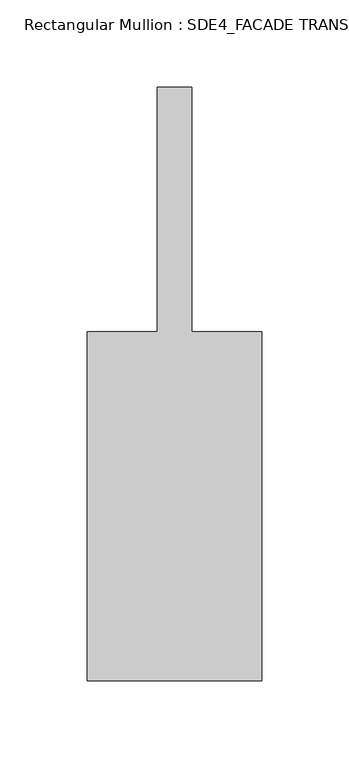
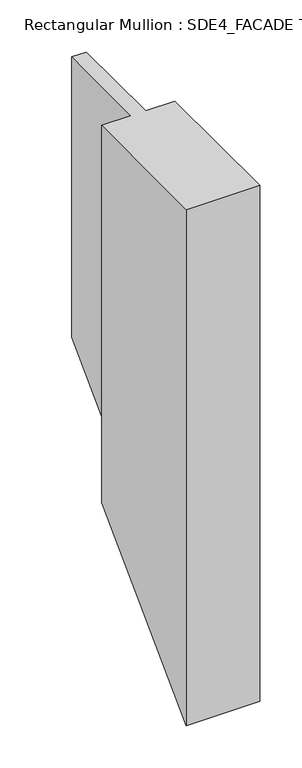
"""IFC4 building model written with IfcOpenShell, lengths in millimetres: member geometry, Rectangular Mullion : SDE4_FACADE TRANSOM TYPE 1."""

from ifc_helpers import new_model, si_unit, origin, place, context, project, spatial, faceted_brep, source, transform, mapped, element, save


def rectangular_mullion_sde4_facade_transom_type_1_dc933e7f(model_context):
    return source(origin(), model_context, "Body", "Brep", [
        faceted_brep([(50.0, -132.5, 0.0), (50.0, 67.5, 0.0), (10.0, 67.5, 0.0), (10.0, 207.5, 0.0), (-10.0, 207.5, 0.0), (-10.0, 67.5, 0.0), (-50.0, 67.5, 0.0), (-50.0, -132.5, 0.0), (50.0, -132.5, -744.0375289), (50.0, 67.5, -544.0375289), (10.0, 67.5, -544.0375289), (10.0, 207.5, -404.0375289), (-10.0, 207.5, -404.0375289), (-10.0, 67.5, -544.0375289), (-50.0, 67.5, -544.0375289), (-50.0, -132.5, -744.0375289)], [[[0, 1, 2, 3, 4, 5, 6, 7]], [[1, 0, 8, 9]], [[2, 1, 9, 10]], [[3, 2, 10, 11]], [[4, 3, 11, 12]], [[5, 4, 12, 13]], [[6, 5, 13, 14]], [[7, 6, 14, 15]], [[0, 7, 15, 8]], [[8, 15, 14, 13, 12, 11, 10, 9]]]),
    ])


if __name__ == "__main__":
    model = new_model("IFC4")
    model_context = context("Model", 3, world=origin())
    ifc_project = project(units=[si_unit("LENGTHUNIT", "METRE", prefix="MILLI")], contexts=[model_context])
    site = spatial("IfcSite", under=ifc_project)
    building = spatial("IfcBuilding", under=site)
    placement = place(None, origin())
    rectangular_mullion_sde4_facade_transom_type_1_shape = rectangular_mullion_sde4_facade_transom_type_1_dc933e7f(model_context)
    element("IfcMember", 1, ObjectType="Rectangular Mullion : SDE4_FACADE TRANSOM TYPE 1", at=placement, inside=building, context=model_context, shape_type="MappedRepresentation", body=[
        mapped(rectangular_mullion_sde4_facade_transom_type_1_shape, transform((0.0, 0.0, 0.0), x_axis=(1.0, 0.0, 0.0), y_axis=(0.0, 1.0, 0.0), z_axis=(0.0, 0.0, 1.0))),
    ])
    save(model, "model.ifc")

# Revit data of these elements
# Type "Rectangular Mullion : SDE4_FACADE TRANSOM TYPE 1"
#   built-in parameter 1007322 = 1.11549 (stored number, unit not read)
#   built-in parameter 1007321 = 0.164042 (stored number, unit not read)
#   built-in parameter 1007320 = 0.164042 (stored number, unit not read)
